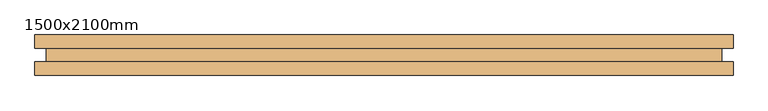
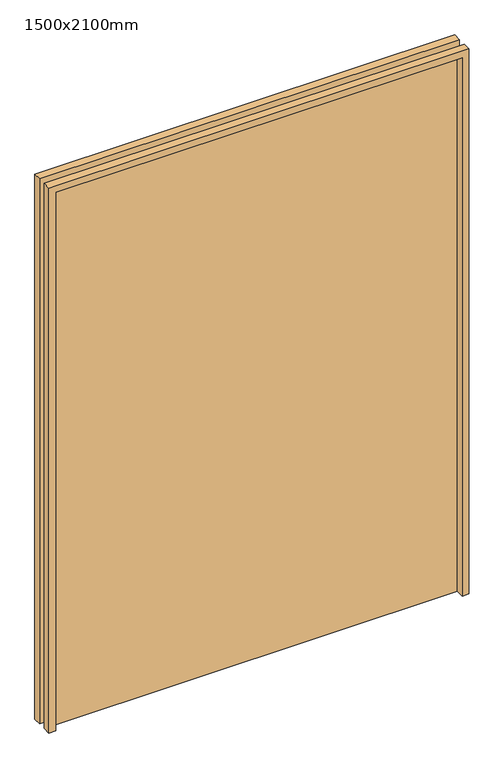
"""IFC4 building model written with IfcOpenShell, lengths in millimetres: door geometry, WWm-SingleSolid-Flush : 1500x2100mm."""

from ifc_helpers import new_model, si_unit, frame, origin, origin_with_axes, place, context, project, spatial, polyline, outline, extrude, source, transform, mapped, element, save


def door_1500x2100mm_f10adb27(model_context):
    return source(origin(), model_context, "Body", "SweptSolid", [
        extrude(outline(polyline([(2125.0, -775.0), (0.0, -775.0), (0.0, -750.0), (2100.0, -750.0), (2100.0, 750.0), (0.0, 750.0), (0.0, 775.0), (2125.0, 775.0), (2125.0, -775.0)])), frame((0.0, -45.0, 0.0), z_axis=(0.0, 1.0, 0.0), x_axis=(0.0, 0.0, 1.0)), (0.0, 0.0, 1.0), 30.0),
        extrude(outline(polyline([(2125.0, 775.0), (2125.0, -775.0), (0.0, -775.0), (0.0, -750.0), (2100.0, -750.0), (2100.0, 750.0), (0.0, 750.0), (0.0, 775.0), (2125.0, 775.0)])), frame((0.0, 15.0, 0.0), z_axis=(0.0, 1.0, 0.0), x_axis=(0.0, 0.0, 1.0)), (0.0, 0.0, 1.0), 30.0),
        extrude(outline(polyline([(750.0, 35.0), (750.0, -15.0), (-750.0, -15.0), (-750.0, 35.0), (750.0, 35.0)])), origin_with_axes(), (0.0, 0.0, 1.0), 2100.0),
    ])


if __name__ == "__main__":
    model = new_model("IFC4")
    model_context = context("Model", 3, world=origin())
    ifc_project = project(units=[si_unit("LENGTHUNIT", "METRE", prefix="MILLI")], contexts=[model_context])
    site = spatial("IfcSite", under=ifc_project)
    building = spatial("IfcBuilding", under=site)
    placement = place(None, origin())
    door_1500x2100mm_shape = door_1500x2100mm_f10adb27(model_context)
    element("IfcDoor", 1, ObjectType="WWm-SingleSolid-Flush : 1500x2100mm", at=placement, inside=building, context=model_context, shape_type="MappedRepresentation", body=[
        mapped(door_1500x2100mm_shape, transform((0.0, 0.0, 0.0), x_axis=(1.0, 0.0, 0.0), y_axis=(0.0, 1.0, 0.0), z_axis=(0.0, 0.0, 1.0))),
    ])
    save(model, "model.ifc")

# Revit data of these elements
# Type "WWm-SingleSolid-Flush : 1500x2100mm"
#   Type Mark = "EX1-58"
#   Construction Type Id = "MDOOR"
#   Assembly Code = "C1020"
#   Analytic Construction = "Metal"
#   Thickness = 50 mm
#   Thermal Resistance (R) = 0.270117 (m²·K)/W
#   Heat Transfer Coefficient (U) = 3.7021 W/(m²·K)
#   Height = 2100 mm
#   Trim Projection Ext = 30 mm
#   Trim Projection Int = 30 mm
#   Trim Width = 25 mm
#   Width = 1500 mm
#   Not 90 Degree [instance default] = no
#   90 Degree [instance default] = yes
#   Door Material = WW-EC-RGB-White
#   Frame Material = WW-EC-RGB-White
#   Visual Light Transmittance = 0
#   Solar Heat Gain Coefficient = 0
#   Function = (empty or 0)
#   Wall Closure = (empty or 0)
# Element 1 (IfcDoor, "WWm-SingleSolid-Flush : 1500x2100mm")
#   Materials on its faces: "WW-EC-RGB-White"
# Materials
#   "WW-EC-RGB-White": class "Generic", colour RGB 255 255 255, transparency 0, Comments = "If region requests off-white, swith asset color to RGB 231-228-220", Description = "Generic Color", Cost = 0
